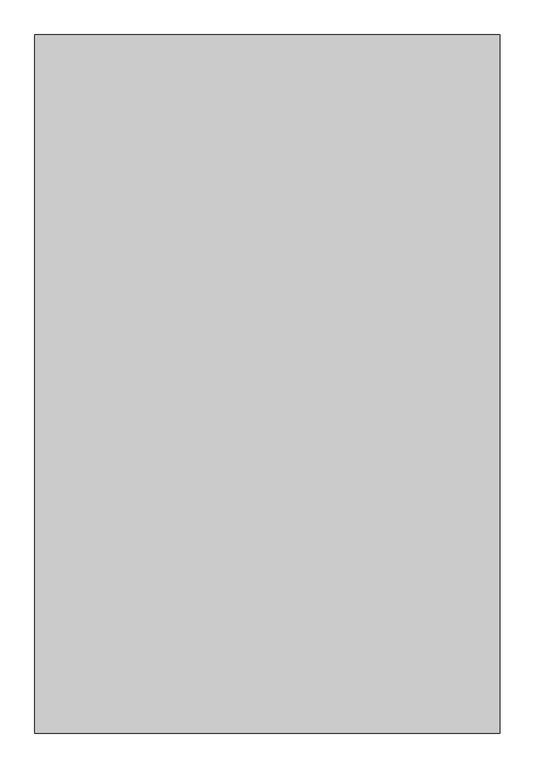
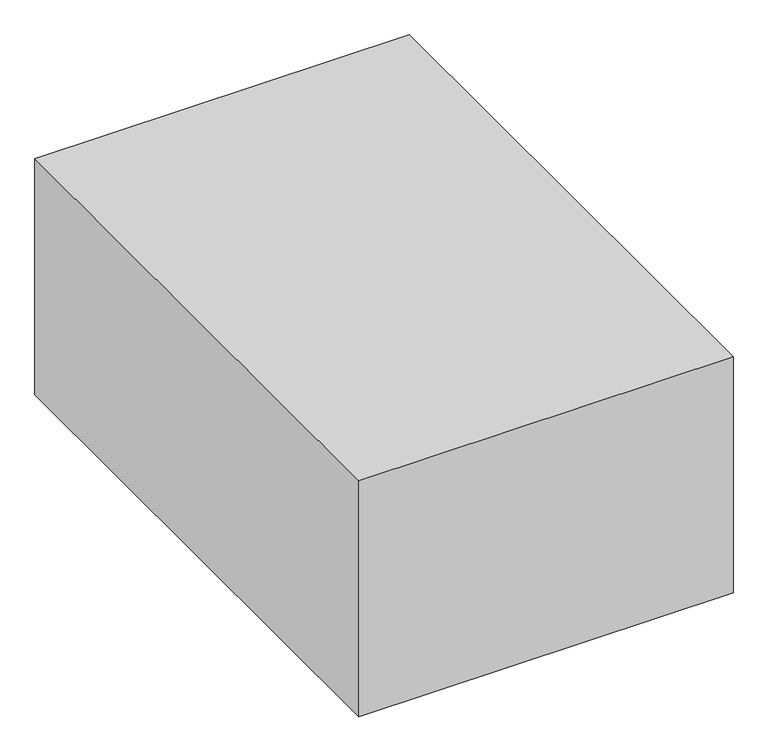
"""IFC4 building model written with IfcOpenShell, lengths in millimetres: proxy geometry, Space Planning Box_hec : Space Planning Box_hec."""

from ifc_helpers import new_model, si_unit, origin, origin_with_axes, place, context, project, spatial, polyline, outline, extrude, source, transform, mapped, element, save


def generic_models_df3bc381(model_context):
    return source(origin(), model_context, "Body", "SweptSolid", [
        extrude(outline(polyline([(4500.0, 6750.0), (4500.0, -6750.0), (-4500.0, -6750.0), (-4500.0, 6750.0), (4500.0, 6750.0)])), origin_with_axes(), (0.0, 0.0, 1.0), 6000.0),
    ])


if __name__ == "__main__":
    model = new_model("IFC4")
    model_context = context("Model", 3, world=origin())
    ifc_project = project(units=[si_unit("LENGTHUNIT", "METRE", prefix="MILLI")], contexts=[model_context])
    site = spatial("IfcSite", under=ifc_project)
    building = spatial("IfcBuilding", under=site)
    placement = place(None, origin())
    generic_models_shape = generic_models_df3bc381(model_context)
    element("IfcBuildingElementProxy", 1, Name="Space Planning Box_hec : Space Planning Box_hec", ObjectType="Space Planning Box_hec : Space Planning Box_hec", at=placement, inside=building, context=model_context, shape_type="MappedRepresentation", body=[
        mapped(generic_models_shape, transform((0.0, 0.0, 0.0), x_axis=(1.0, 0.0, 0.0), y_axis=(0.0, 1.0, 0.0), z_axis=(0.0, 0.0, 1.0))),
    ])
    save(model, "model.ifc")

# Revit data of these elements
# Type "Space Planning Box_hec : Space Planning Box_hec"
#   Type Comments = "..."
#   Room Name [instance default] = "?"
#   Interior Finish [instance default] = ""
#   Exterior Finish [instance default] = ""
#   Department [instance default] = ""
#   Assembly Code = "..."
#   Width [instance default] = 1524 mm
#   Program Area [instance default] = 0.00 m²
#   Length [instance default] = 1524 mm
#   Height [instance default] = 1524 mm
#   Area [instance default] = 2.32258 m²
#   Fill Color [instance default] = Cyan
#   Default Elevation = 0
# Element 1 (IfcBuildingElementProxy, "Space Planning Box_hec : Space Planning Box_hec")
#   Room Name = "Engineer Room"
#   Interior Finish = "IF3"
#   Exterior Finish = "EF1"
#   Department = "CI"
#   Width = 9000 mm
#   Program Area = 120.00 m²
#   Length = 13500 mm
#   Height = 6000 mm
#   Area = 121.50 m²
#   Fill Color = Lime
#   Materials on its faces: "Lime"
# Materials
#   "Cyan": class "Generic", colour RGB 0 255 255, transparency 0.2, Cost = 0
#   "Lime": class "Generic", colour RGB 0 255 0, transparency 0.2, Cost = 0
